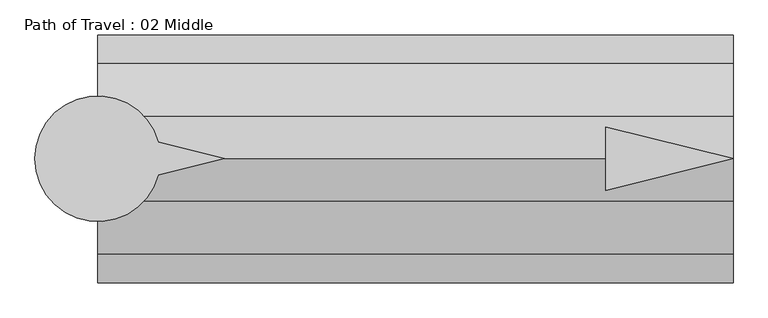
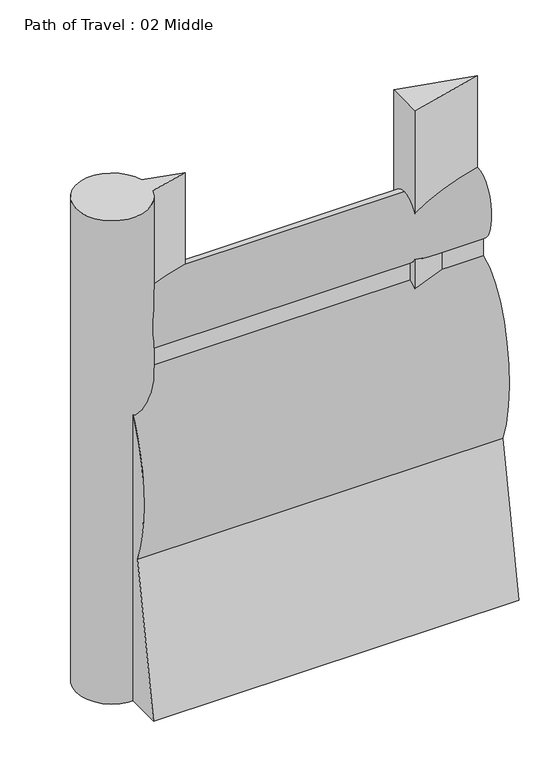
"""IFC4 building model written with IfcOpenShell, lengths in millimetres: proxy geometry, Path of Travel : 02 Middle."""

import ifcopenshell
import ifcopenshell.guid

model = None  # the IFC model being written
_history = None  # IfcOwnerHistory: only IFC2X3 demands one
_inside = {}  # id of a spatial element -> (the spatial element, [elements in it])
_under = {}  # id of a project, library or spatial element -> (it, [spatial elements below it])
_declared = {}  # id of a project -> (the project, [libraries it declares])
_typed = {}  # id of a type object -> (the type object, [elements of that type])
_made_of = {}  # id of a material, layer set ... -> (it, [elements and type objects made of it])


def new_model(schema):
    """Start an empty IFC model of exactly this schema.

    Asked for "IFC4X3", IfcOpenShell would pick the latest addendum, in which some entities
    have other attributes; the version numbers below select the first issue.
    IFC2X3 requires an IfcOwnerHistory on every rooted entity: one is made here for all.
    """
    global model, _history
    if schema == "IFC4X3":
        model = ifcopenshell.file(schema_version=(4, 3, 0, 0))
    else:
        model = ifcopenshell.file(schema=schema)
    _inside.clear()
    _under.clear()
    _declared.clear()
    _typed.clear()
    _made_of.clear()
    _history = None
    if model.schema == "IFC2X3":
        org = make("IfcOrganization", Name="unknown")
        user = make(
            "IfcPersonAndOrganization",
            ThePerson=make("IfcPerson", FamilyName="unknown"),
            TheOrganization=org,
        )
        app = make(
            "IfcApplication",
            ApplicationDeveloper=org,
            Version="unknown",
            ApplicationFullName="unknown",
            ApplicationIdentifier="unknown",
        )
        _history = make(
            "IfcOwnerHistory",
            OwningUser=user,
            OwningApplication=app,
            ChangeAction="ADDED",
            CreationDate=0,
        )
    return model


def make(cls, **values):
    """One entity of the class cls with the attributes given. An attribute that is None is left unset."""
    return model.create_entity(
        cls, **{name: value for name, value in values.items() if value is not None}
    )


def rooted(cls, **values):
    """An entity with a GlobalId (a new one), such as an element, a storey or a relation."""
    return make(cls, GlobalId=ifcopenshell.guid.new(), OwnerHistory=_history, **values)


def si_unit(unit_type, name, prefix=None):
    """IfcSIUnit, for example si_unit("LENGTHUNIT", "METRE", prefix="MILLI")."""
    return make("IfcSIUnit", UnitType=unit_type, Prefix=prefix, Name=name)


def assignment(units):
    """IfcUnitAssignment: the units of a project."""
    return None if units is None else make("IfcUnitAssignment", Units=units)


def point(xyz):
    """IfcCartesianPoint."""
    return None if xyz is None else make("IfcCartesianPoint", Coordinates=xyz)


def direction(xyz):
    """IfcDirection."""
    return None if xyz is None else make("IfcDirection", DirectionRatios=xyz)


def frame(location, z_axis=None, x_axis=None):
    """IfcAxis2Placement3D, a coordinate frame: its origin and axes. An axis left out is left unset."""
    return make(
        "IfcAxis2Placement3D",
        Location=point(location),
        Axis=direction(z_axis),
        RefDirection=direction(x_axis),
    )


def frame_2d(location, x_axis=None):
    """IfcAxis2Placement2D, a coordinate frame in the plane: its origin and x axis."""
    return make(
        "IfcAxis2Placement2D", Location=point(location), RefDirection=direction(x_axis)
    )


def origin():
    """The frame at (0, 0, 0) with its axes left unset."""
    return frame((0.0, 0.0, 0.0))


def origin_with_axes():
    """The frame at (0, 0, 0) with the z axis (0, 0, 1) and the x axis (1, 0, 0) written out."""
    return frame((0.0, 0.0, 0.0), z_axis=(0.0, 0.0, 1.0), x_axis=(1.0, 0.0, 0.0))


def place(relative_to, where):
    """IfcLocalPlacement: puts the frame where relative to a parent placement (None: the world)."""
    return make(
        "IfcLocalPlacement", PlacementRelTo=relative_to, RelativePlacement=where
    )


def context(
    kind, dimensions, precision=None, world=None, true_north=None, identifier=None
):
    """IfcGeometricRepresentationContext, for example the 3D "Model" context."""
    return make(
        "IfcGeometricRepresentationContext",
        ContextIdentifier=identifier,
        ContextType=kind,
        CoordinateSpaceDimension=dimensions,
        Precision=precision,
        WorldCoordinateSystem=world,
        TrueNorth=true_north,
    )


def project(units=None, contexts=None):
    """IfcProject with its units and contexts."""
    return rooted(
        "IfcProject",
        Name="project",
        RepresentationContexts=contexts,
        UnitsInContext=assignment(units),
    )


def spatial(cls, under=None, at=None, **own):
    """A site, building, storey or space (cls), placed at a placement, below another one or the project."""
    s = rooted(cls, ObjectPlacement=at, **own)
    if under is not None:
        _under.setdefault(under.id(), (under, []))[1].append(s)
    return s


def polyline(points):
    """IfcPolyline through the points."""
    return make("IfcPolyline", Points=[point(p) for p in points])


def circle_curve(where, radius):
    """IfcCircle in the frame where."""
    return make("IfcCircle", Position=where, Radius=radius)


def ellipse_curve(where, semi_axis1, semi_axis2):
    """IfcEllipse in the frame where."""
    return make(
        "IfcEllipse", Position=where, SemiAxis1=semi_axis1, SemiAxis2=semi_axis2
    )


def trimmed(basis, trim1, trim2, sense, master):
    """IfcTrimmedCurve: the piece of a basis curve between two trims."""
    return make(
        "IfcTrimmedCurve",
        BasisCurve=basis,
        Trim1=trim1,
        Trim2=trim2,
        SenseAgreement=sense,
        MasterRepresentation=master,
    )


def segment(curve, same_sense, transition):
    """IfcCompositeCurveSegment."""
    return make(
        "IfcCompositeCurveSegment",
        Transition=transition,
        SameSense=same_sense,
        ParentCurve=curve,
    )


def composite_curve(segments, self_intersect=None):
    """IfcCompositeCurve: segments joined end to end."""
    return make("IfcCompositeCurve", Segments=segments, SelfIntersect=self_intersect)


def outline(outer, holes=None, kind="AREA"):
    """IfcArbitraryClosedProfileDef: a profile drawn as a closed curve; with holes, ...WithVoids."""
    if holes is None:
        return make("IfcArbitraryClosedProfileDef", ProfileType=kind, OuterCurve=outer)
    return make(
        "IfcArbitraryProfileDefWithVoids",
        ProfileType=kind,
        OuterCurve=outer,
        InnerCurves=holes,
    )


def extrude(swept, where, along, depth):
    """IfcExtrudedAreaSolid: the profile swept, set in the frame where, extruded along a direction by depth."""
    return make(
        "IfcExtrudedAreaSolid",
        SweptArea=swept,
        Position=where,
        ExtrudedDirection=direction(along),
        Depth=depth,
    )


def shape(context_of_items, identifier, shape_type, items):
    """IfcShapeRepresentation: the items that make up one representation, for example the "Body"."""
    return make(
        "IfcShapeRepresentation",
        ContextOfItems=context_of_items,
        RepresentationIdentifier=identifier,
        RepresentationType=shape_type,
        Items=items,
    )


def source(mapping_origin, context_of_items, identifier, shape_type, items):
    """IfcRepresentationMap: a shape defined once, which mapped items show again and again."""
    return make(
        "IfcRepresentationMap",
        MappingOrigin=mapping_origin,
        MappedRepresentation=shape(context_of_items, identifier, shape_type, items),
    )


def transform(
    local_origin,
    x_axis=None,
    y_axis=None,
    z_axis=None,
    scale=None,
    scale2=None,
    scale3=None,
    uniform=True,
):
    """IfcCartesianTransformationOperator3D, or its non-uniform kind. x_axis, y_axis, z_axis: its Axis1, 2, 3."""
    if uniform:
        return make(
            "IfcCartesianTransformationOperator3D",
            Axis1=direction(x_axis),
            Axis2=direction(y_axis),
            LocalOrigin=point(local_origin),
            Scale=scale,
            Axis3=direction(z_axis),
        )
    return make(
        "IfcCartesianTransformationOperator3DnonUniform",
        Axis1=direction(x_axis),
        Axis2=direction(y_axis),
        LocalOrigin=point(local_origin),
        Scale=scale,
        Axis3=direction(z_axis),
        Scale2=scale2,
        Scale3=scale3,
    )


def mapped(mapping_source, mapping_target):
    """IfcMappedItem: shows the shape of a source again, moved by a transform."""
    return make(
        "IfcMappedItem", MappingSource=mapping_source, MappingTarget=mapping_target
    )


def made_of(thing, what):
    """Note that an element or type object is made of a material, layer set ...; save() writes the relation."""
    if what is not None:
        _made_of.setdefault(what.id(), (what, []))[1].append(thing)
    return thing


def element(
    cls,
    number,
    at=None,
    inside=None,
    cuts=None,
    type_object=None,
    material=None,
    context=None,
    identifier="Body",
    shape_type=None,
    held_by="IfcProductDefinitionShape",
    body=None,
    shapes=None,
    **own,
):
    """One element of the class cls, such as IfcWall. Its Tag is "e" and its number.

    at: its placement. inside: the storey or other place that contains it. cuts: it is an
    opening in that element (IfcRelVoidsElement). A single representation is given by context,
    identifier, shape_type and body (its items); several are given by shapes. held_by: the class
    of the entity that holds the representations. save() writes the other relations.
    """
    e = rooted(cls, Tag="e%d" % number, ObjectPlacement=at, **own)
    if body is not None:
        shapes = [shape(context, identifier, shape_type, body)]
    if shapes is not None:
        e.Representation = make(held_by, Representations=shapes)
    if inside is not None:
        _inside.setdefault(inside.id(), (inside, []))[1].append(e)
    if cuts is not None:
        rooted(
            "IfcRelVoidsElement", RelatingBuildingElement=cuts, RelatedOpeningElement=e
        )
    if type_object is not None:
        _typed.setdefault(type_object.id(), (type_object, []))[1].append(e)
    return made_of(e, material)


def aggregate(whole, parts):
    """IfcRelAggregates: a whole, such as a stair, and the parts it consists of."""
    return rooted("IfcRelAggregates", RelatingObject=whole, RelatedObjects=parts)


def save(model, path):
    """Write the relations noted so far, then the file.

    IfcRelAggregates (storeys below a building ...), IfcRelContainedInSpatialStructure (elements
    in a storey), IfcRelDefinesByType, IfcRelAssociatesMaterial and IfcRelDeclares: one each for
    every whole, place, type object, material and project.
    """
    for whole, parts in _under.values():
        aggregate(whole, parts)
    for where, things in _inside.values():
        rooted(
            "IfcRelContainedInSpatialStructure",
            RelatedElements=things,
            RelatingStructure=where,
        )
    for kind, things in _typed.values():
        rooted("IfcRelDefinesByType", RelatedObjects=things, RelatingType=kind)
    for what, things in _made_of.values():
        rooted("IfcRelAssociatesMaterial", RelatedObjects=things, RelatingMaterial=what)
    for by, libraries in _declared.values():
        rooted("IfcRelDeclares", RelatingContext=by, RelatedDefinitions=libraries)
    model.write(path)


def plane_surface(at):
    """IfcPlane: the flat surface through the origin of the frame at, square to its z axis."""
    return make("IfcPlane", Position=at)


def extruded_surface(curve, direction_of_extrusion, depth):
    """IfcSurfaceOfLinearExtrusion: the curve pushed along a direction by depth."""
    return make(
        "IfcSurfaceOfLinearExtrusion",
        SweptCurve=make("IfcArbitraryOpenProfileDef", ProfileType="CURVE", Curve=curve),
        ExtrudedDirection=direction(direction_of_extrusion),
        Depth=depth,
    )


def advanced_brep(points, edges, surfaces, faces):
    """IfcAdvancedBrep: a solid bounded by faces that lie on surfaces and meet in shared edges.

    An edge is (start, end): straight between two places in points (the first is 0);
    or (start, end, curve); or (start, end, curve, False) where it runs against its curve.
    A face is (place in surfaces, loops), or (place, loops, False) where it looks against
    its surface's normal. A loop lists edges by number (the first is 1), with a minus sign
    where the edge is run from its end to its start. The first loop is the outer one.
    """
    corners = [point(p) for p in points]
    vertices = [make("IfcVertexPoint", VertexGeometry=c) for c in corners]
    made = []
    for start, end, *more in edges:
        made.append(
            make(
                "IfcEdgeCurve",
                EdgeStart=vertices[start],
                EdgeEnd=vertices[end],
                EdgeGeometry=more[0] if more else make("IfcPolyline", Points=[corners[start], corners[end]]),
                SameSense=more[1] if len(more) > 1 else True,
            )
        )
    hull = []
    for where, loops, *sense in faces:
        bounds = []
        for j, loop in enumerate(loops):
            ring = [make("IfcOrientedEdge", EdgeElement=made[abs(k) - 1], Orientation=k > 0) for k in loop]
            bounds.append(
                make(
                    "IfcFaceOuterBound" if j == 0 else "IfcFaceBound",
                    Bound=make("IfcEdgeLoop", EdgeList=ring),
                    Orientation=True,
                )
            )
        hull.append(make("IfcAdvancedFace", Bounds=bounds, FaceSurface=surfaces[where], SameSense=sense[0] if sense else True))
    return make("IfcAdvancedBrep", Outer=make("IfcClosedShell", CfsFaces=hull))


def path_of_travel_02_middle_987670bd(model_context):
    return source(origin(), model_context, "Body", "SolidModel", [
        advanced_brep(
        [(227.5554837, 0.0, 1727.2), (227.5554837, 42.9018657, 1436.6534209), (227.5554837, 42.9018657, 1363.4763406), (227.5554837, 184.1186263, 643.4144547), (227.5554837, 297.5699544, 0.0), (227.5554837, 145.6574193, 0.0), (227.5554837, 0.0, 584.2), (227.5554837, -145.6574193, 0.0), (227.5554837, -297.5699544, 0.0), (227.5554837, -184.1186263, 643.4144547), (227.5554837, -42.9018657, 1363.4763406), (227.5554837, -42.9018657, 1436.6534209), (1751.5554837, 0.0, 1727.2), (1751.5554837, -42.9018657, 1436.6534209), (1751.5554837, -42.9018657, 1363.4763406), (1751.5554837, -184.1186263, 643.4144547), (1751.5554837, -297.5699544, 0.0), (1751.5554837, -145.6574193, 0.0), (1751.5554837, 0.0, 584.2), (1751.5554837, 145.6574193, 0.0), (1751.5554837, 297.5699544, 0.0), (1751.5554837, 184.1186263, 643.4144547), (1751.5554837, 42.9018657, 1363.4763406), (1751.5554837, 42.9018657, 1436.6534209)],
        [
            (0, 1, ellipse_curve(frame((227.5554837, 0.0, 1574.8), z_axis=(-1.0, 0.0, 0.0), x_axis=(0.0, 0.0, 1.0)), 152.4, 101.6)),
            (1, 2),
            (2, 3, ellipse_curve(frame((227.5554837, 0.0, 914.4), z_axis=(-1.0, 0.0, 0.0), x_axis=(0.0, 0.0, -1.0)), 457.2, 228.6)),
            (3, 4),
            (4, 5),
            (5, 6),
            (6, 7),
            (7, 8),
            (8, 9),
            (9, 10, ellipse_curve(frame((227.5554837, 0.0, 914.4), z_axis=(-1.0, 0.0, 0.0), x_axis=(0.0, 0.0, -1.0)), 457.2, 228.6)),
            (10, 11),
            (11, 0, ellipse_curve(frame((227.5554837, 0.0, 1574.8), z_axis=(-1.0, 0.0, 0.0), x_axis=(0.0, 0.0, 1.0)), 152.4, 101.6)),
            (12, 13, ellipse_curve(frame((1751.5554837, 0.0, 1574.8), z_axis=(1.0, 0.0, 0.0), x_axis=(0.0, 0.0, 1.0)), 152.4, 101.6)),
            (13, 14),
            (14, 15, ellipse_curve(frame((1751.5554837, 0.0, 914.4), z_axis=(1.0, 0.0, 0.0), x_axis=(0.0, 0.0, -1.0)), 457.2, 228.6)),
            (15, 16),
            (16, 17),
            (17, 18),
            (18, 19),
            (19, 20),
            (20, 21),
            (21, 22, ellipse_curve(frame((1751.5554837, 0.0, 914.4), z_axis=(1.0, 0.0, 0.0), x_axis=(0.0, 0.0, -1.0)), 457.2, 228.6)),
            (22, 23),
            (23, 12, ellipse_curve(frame((1751.5554837, 0.0, 1574.8), z_axis=(1.0, 0.0, 0.0), x_axis=(0.0, 0.0, 1.0)), 152.4, 101.6)),
            (0, 12),
            (23, 1),
            (22, 2),
            (21, 3),
            (20, 4),
            (19, 5),
            (18, 6),
            (17, 7),
            (16, 8),
            (15, 9),
            (14, 10),
            (13, 11),
        ],
        [
            plane_surface(frame((227.5554837, 0.0, 0.0), z_axis=(-1.0, 0.0, 0.0), x_axis=(0.0, 0.0, 1.0))),
            plane_surface(frame((1751.5554837, 0.0, 0.0), z_axis=(1.0, 0.0, 0.0), x_axis=(0.0, 0.0, 1.0))),
            extruded_surface(trimmed(ellipse_curve(frame((1751.5554837, 0.0, 1574.8), z_axis=(-1.0, 0.0, 0.0), x_axis=(0.0, 0.0, 1.0)), 152.4, 101.6), [point((1751.5554837, 0.0, 1727.2))], [point((1751.5554837, 42.9018657, 1436.6534209))], True, "CARTESIAN"), (-1524.0, 0.0, 0.0), 1524.0),
            plane_surface(frame((227.5554837, 42.9018657, 1436.6534209), z_axis=(0.0, 1.0, 0.0), x_axis=(1.0, 0.0, 0.0))),
            extruded_surface(trimmed(ellipse_curve(frame((1751.5554837, 0.0, 914.4), z_axis=(-1.0, 0.0, 0.0), x_axis=(0.0, 0.0, -1.0)), 457.2, 228.6), [point((1751.5554837, 42.9018657, 1363.4763406))], [point((1751.5554837, 184.1186263, 643.4144547))], True, "CARTESIAN"), (-1524.0, 0.0, 0.0), 1524.0),
            plane_surface(frame((227.5554837, 184.1186263, 643.4144547), z_axis=(0.0, 0.9848077530122078, 0.1736481776669322), x_axis=(1.0, 0.0, 0.0))),
            plane_surface(frame((227.5554837, 297.5699544, 0.0), z_axis=(0.0, 0.0, -1.0), x_axis=(1.0, 0.0, 0.0))),
            plane_surface(frame((227.5554837, 145.6574193, 0.0), z_axis=(0.0, -0.9702957262760199, -0.2419218955995739), x_axis=(1.0, 0.0, 0.0))),
            plane_surface(frame((227.5554837, 0.0, 584.2), z_axis=(0.0, 0.9702957262759961, -0.24192189559966923), x_axis=(1.0, 0.0, 0.0))),
            plane_surface(frame((227.5554837, -145.6574193, 0.0), z_axis=(0.0, 0.0, -1.0), x_axis=(1.0, 0.0, 0.0))),
            plane_surface(frame((227.5554837, -297.5699544, 0.0), z_axis=(0.0, -0.984807753012208, 0.17364817766693066), x_axis=(1.0, 0.0, 0.0))),
            extruded_surface(trimmed(ellipse_curve(frame((1751.5554837, 0.0, 914.4), z_axis=(-1.0, 0.0, 0.0), x_axis=(0.0, 0.0, -1.0)), 457.2, 228.6), [point((1751.5554837, -184.1186263, 643.4144547))], [point((1751.5554837, -42.9018657, 1363.4763406))], True, "CARTESIAN"), (-1524.0, 0.0, 0.0), 1524.0),
            plane_surface(frame((227.5554837, -42.9018657, 1363.4763406), z_axis=(0.0, -1.0, 0.0), x_axis=(1.0, 0.0, 0.0))),
            extruded_surface(trimmed(ellipse_curve(frame((1751.5554837, 0.0, 1574.8), z_axis=(-1.0, 0.0, 0.0), x_axis=(0.0, 0.0, 1.0)), 152.4, 101.6), [point((1751.5554837, -42.9018657, 1436.6534209))], [point((1751.5554837, 0.0, 1727.2))], True, "CARTESIAN"), (-1524.0, 0.0, 0.0), 1524.0),
        ],
        [
            (0, [[1, 2, 3, 4, 5, 6, 7, 8, 9, 10, 11, 12]]),
            (1, [[13, 14, 15, 16, 17, 18, 19, 20, 21, 22, 23, 24]]),
            (2, [[-1, 25, -24, 26]]),
            (3, [[-2, -26, -23, 27]]),
            (4, [[-3, -27, -22, 28]]),
            (5, [[-4, -28, -21, 29]]),
            (6, [[-5, -29, -20, 30]]),
            (7, [[-6, -30, -19, 31]]),
            (8, [[-7, -31, -18, 32]]),
            (9, [[-8, -32, -17, 33]]),
            (10, [[-9, -33, -16, 34]]),
            (11, [[-10, -34, -15, 35]]),
            (12, [[-11, -35, -14, 36]]),
            (13, [[-12, -36, -13, -25]]),
        ],
    ),
        extrude(outline(polyline([(1445.5503371, 76.2006338), (1751.5554837, 0.0), (1445.5503371, -76.2006338), (1445.5503371, 76.2006338)])), origin_with_axes(), (0.0, 0.0, 1.0), 2129.5973753),
        extrude(outline(composite_curve([segment(polyline([(372.7837828, 39.4440225), (531.182385, 0.0), (372.7837828, -39.4440225)]), True, "CONTINUOUS"), segment(trimmed(circle_curve(frame_2d((227.2200886, 0.0)), 150.8131956), [point((372.7837828, -39.4440225))], [point((372.7837828, 39.4440225))], False, "CARTESIAN"), True, "CONTINUOUS")], self_intersect=False)), origin_with_axes(), (0.0, 0.0, 1.0), 2129.5973753),
    ])


if __name__ == "__main__":
    model = new_model("IFC4")
    model_context = context("Model", 3, world=origin())
    ifc_project = project(units=[si_unit("LENGTHUNIT", "METRE", prefix="MILLI")], contexts=[model_context])
    site = spatial("IfcSite", under=ifc_project)
    building = spatial("IfcBuilding", under=site)
    placement = place(None, origin())
    path_of_travel_02_middle_shape = path_of_travel_02_middle_987670bd(model_context)
    element("IfcBuildingElementProxy", 1, Name="Path of Travel : 02 Middle", ObjectType="Path of Travel : 02 Middle", at=placement, inside=building, context=model_context, shape_type="MappedRepresentation", body=[
        mapped(path_of_travel_02_middle_shape, transform((0.0, 0.0, 0.0), x_axis=(1.0, 0.0, 0.0), y_axis=(0.0, 1.0, 0.0), z_axis=(0.0, 0.0, 1.0))),
    ])
    save(model, "model.ifc")

# Revit data of these elements
# Type "Path of Travel : 02 Middle"
#   Path of Egress [instance default] = 4' - 0"
#   built-in parameter 1001306 [instance default] = 4 (stored number, unit not read)
#   Dot at Start = no
#   Arrow in Middle = yes
#   Arrow at End = no
#   Egress Path = none
# Element 1 (IfcBuildingElementProxy, "Path of Travel : 02 Middle")
#   Path of Egress = 5' - 0"
#   built-in parameter 1001306 = 5 (stored number, unit not read)
#   Materials on its faces: "Egress Path Solid", "solid"
# Materials
#   "Egress Path Solid": class "Unassigned", colour RGB 255 128 64, transparency 0.75, Comments = "Rendering appearance not upgraded "
#   "solid": class "Generic", colour RGB 120 120 120, transparency 0, Cost = 0
